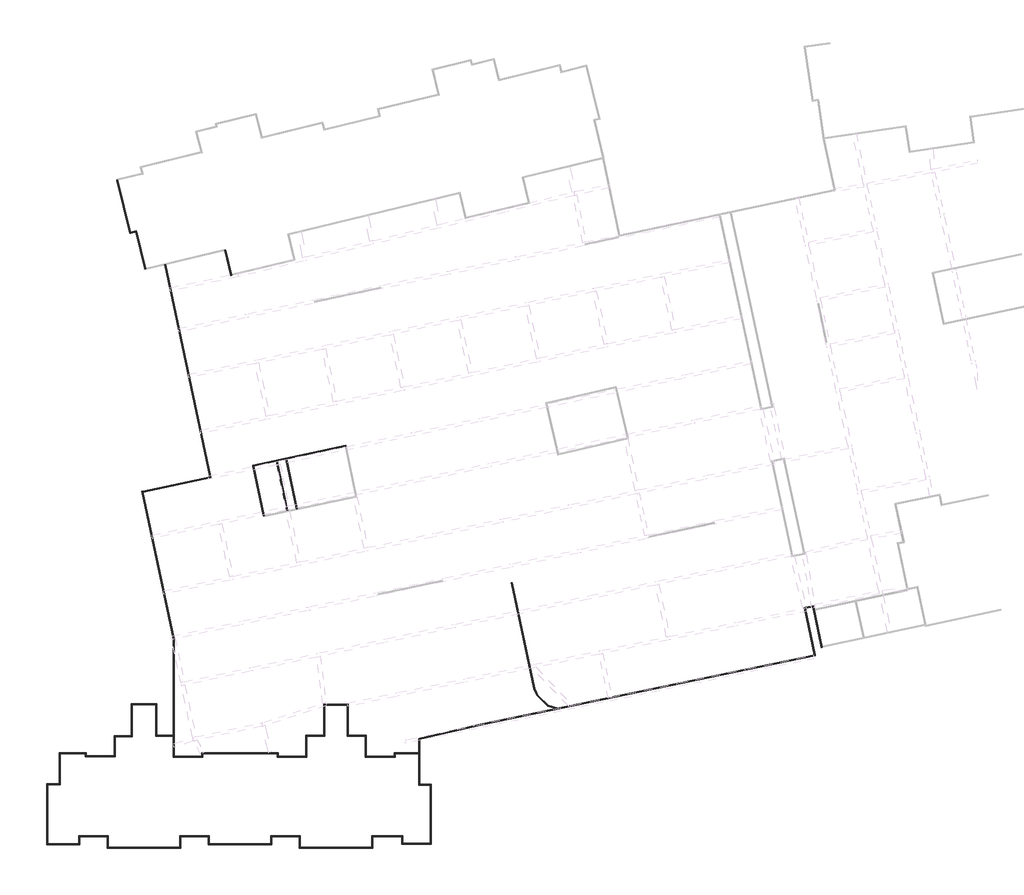
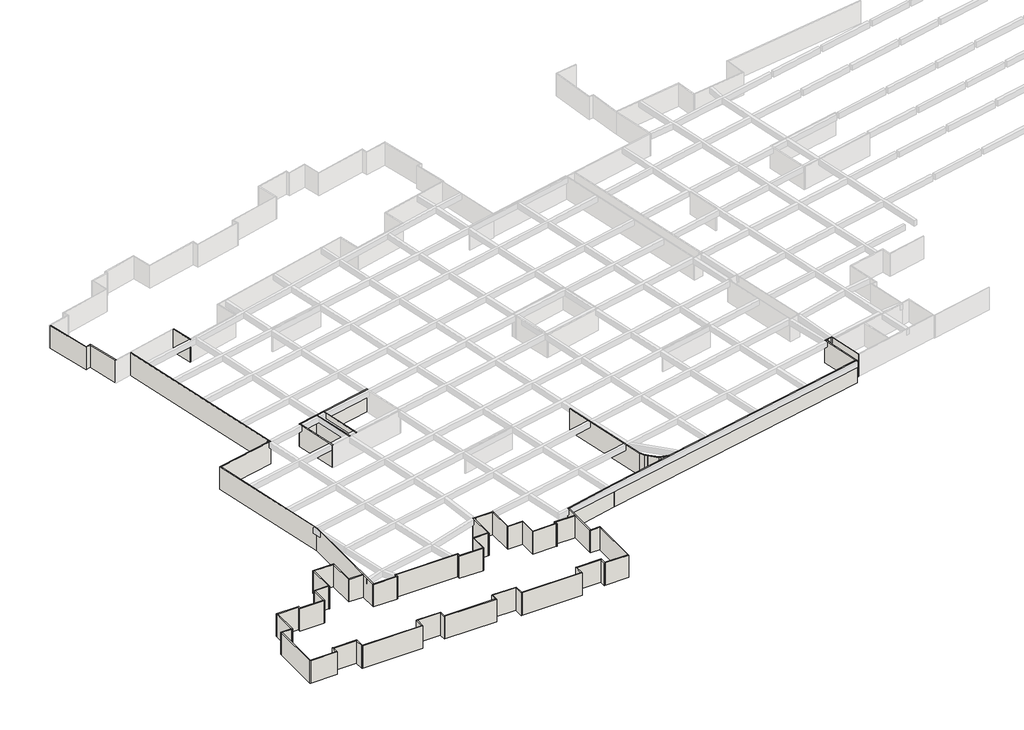
# One storey, part 1 of 14: 68 walls.
# Revit data of these elements (continued)
# Area, not placed, upper offset 0 mm, lower offset 0 mm
#   Number = "24"
#   Name = "fire_compart"
# Area, not placed, upper offset 0 mm, lower offset 0 mm
#   Number = "103"
#   Name = "main_building"
# Area, not placed, upper offset 0 mm, lower offset 0 mm
#   Number = "58"
#   Name = "fire_compart"
# Area, not placed, upper offset 0 mm, lower offset 0 mm
#   Number = "98"
#   Name = "fire_compart"
# Area, not placed, upper offset 0 mm, lower offset 0 mm
#   Number = "99"
#   Name = "main_building"
# Area, not placed, upper offset 0 mm, lower offset 0 mm
#   Number = "123"
#   Name = "main_building"
# Area at (-85290.668, -133064.536) mm, upper offset 0 mm, lower offset 0 mm
#   Number = "172"
#   Name = "fire_compart"
# Area, not placed, upper offset 0 mm, lower offset 0 mm
#   Number = "59"
#   Name = "fire_compart"
# Area at (-332558.106, -211971.491) mm, upper offset 0 mm, lower offset 0 mm
#   Number = "161"
#   Name = "main_building"
# Area at (-320626.882, -142375.996) mm, upper offset 0 mm, lower offset 0 mm
#   Number = "167"
#   Name = "main_building"
# Room, not placed, phase "新构造", upper offset 0 mm, lower offset 0 mm
#   Number = "1"
#   Name = "客餐厅"
# Room, not placed, phase "新构造", upper offset 0 mm, lower offset 0 mm
#   Number = "2"
#   Name = "阳台"
# Room, not placed, phase "新构造", upper offset 0 mm, lower offset 0 mm
#   Number = "3"
#   Name = "次卧"
# Room, not placed, phase "新构造", upper offset 0 mm, lower offset 0 mm
#   Number = "4"
#   Name = "厨房"
# Area, not placed, upper offset 0 mm, lower offset 0 mm
#   Number = "108"
#   Name = "main_building"
# Room, not placed, phase "新构造", upper offset 0 mm, lower offset 0 mm
#   Number = "5"
#   Name = "卫生间"
# Room, not placed, phase "新构造", upper offset 0 mm, lower offset 0 mm
#   Number = "6"
#   Name = "次卧"
# Room, not placed, phase "新构造", upper offset 0 mm, lower offset 0 mm
#   Number = "7"
#   Name = "主卧"
# Area, not placed, upper offset 0 mm, lower offset 0 mm
#   Number = "60"
#   Name = "fire_compart"
# Area, not placed, upper offset 0 mm, lower offset 0 mm
#   Number = "173"
#   Name = "面积"
# Area at (-58171.977, -181534.095) mm, upper offset 0 mm, lower offset 0 mm
#   Number = "174"
#   Name = "fire_compart"
# Area, not placed, upper offset 0 mm, lower offset 0 mm
#   Number = "23"
#   Name = "main_building"
# Area, not placed, upper offset 0 mm, lower offset 0 mm
#   Number = "124"
#   Name = "fire_compart"
# Area, not placed, upper offset 0 mm, lower offset 0 mm
#   Number = "36"
#   Name = "main_building"
# Area, not placed, upper offset 0 mm, lower offset 0 mm
#   Number = "37"
#   Name = "main_building"
# Area, not placed, upper offset 0 mm, lower offset 0 mm
#   Number = "38"
#   Name = "main_building"
# Area, not placed, upper offset 0 mm, lower offset 0 mm
#   Number = "39"
#   Name = "main_building"
# Area, not placed, upper offset 0 mm, lower offset 0 mm
#   Number = "40"
#   Name = "main_building"
# Area, not placed, upper offset 0 mm, lower offset 0 mm
#   Number = "64"
#   Name = "fire_compart"
# Area, not placed, upper offset 0 mm, lower offset 0 mm
#   Number = "61"
#   Name = "fire_compart"
# Area, not placed, upper offset 0 mm, lower offset 0 mm
#   Number = "65"
#   Name = "main_building"
# Area, not placed, upper offset 0 mm, lower offset 0 mm
#   Number = "104"
#   Name = "main_building"
# Area, not placed, upper offset 0 mm, lower offset 0 mm
#   Number = "62"
#   Name = "fire_compart"
# Area, not placed, upper offset 0 mm, lower offset 0 mm
#   Number = "125"
#   Name = "fire_compart"
# Area at (-54639.354, -203766.854) mm, upper offset 0 mm, lower offset 0 mm
#   Number = "164"
#   Name = "main_building"
# Area, not placed, upper offset 0 mm, lower offset 0 mm
#   Number = "63"
#   Name = "fire_compart"
# Area, not placed, upper offset 0 mm, lower offset 0 mm
#   Number = "66"
#   Name = "main_building"
# Area, not placed, upper offset 0 mm, lower offset 0 mm
#   Number = "126"
#   Name = "fire_compart"
# Area, not placed, upper offset 0 mm, lower offset 0 mm
#   Number = "83"
#   Name = "fire_compart"
# Area, not placed, upper offset 0 mm, lower offset 0 mm
#   Number = "84"
#   Name = "main_building"
# Area, not placed, upper offset 0 mm, lower offset 0 mm
#   Number = "150"
#   Name = "main_building"
# Area, not placed, upper offset 0 mm, lower offset 0 mm
#   Number = "127"
#   Name = "fire_compart"
# Area, not placed, upper offset 0 mm, lower offset 0 mm
#   Number = "7"
#   Name = "fire_compart_5"
# Area at (-166160.857, -117669.33) mm, upper offset 0 mm, lower offset 0 mm
#   Number = "175"
#   Name = "main_building"
# Area at (-77453.482, -110613.298) mm, upper offset 0 mm, lower offset 0 mm
#   Number = "176"
#   Name = "main_building"
# Area, not placed, upper offset 0 mm, lower offset 0 mm
#   Number = "128"
#   Name = "fire_compart"
# Area at (-242035.568, -186509.315) mm, upper offset 0 mm, lower offset 0 mm
#   Number = "162"
#   Name = "main_building"
# Area, not placed, upper offset 0 mm, lower offset 0 mm
#   Number = "129"
#   Name = "fire_compart"
# Area, not placed, upper offset 0 mm, lower offset 0 mm
#   Number = "151"
#   Name = "main_building"
# Area, not placed, upper offset 0 mm, lower offset 0 mm
#   Number = "130"
#   Name = "fire_compart"
# Area, not placed, upper offset 0 mm, lower offset 0 mm
#   Number = "109"
#   Name = "main_building"
# Area, not placed, upper offset 0 mm, lower offset 0 mm
#   Number = "67"
#   Name = "fire_compart"
# Area, not placed, upper offset 0 mm, lower offset 0 mm
#   Number = "112"
#   Name = "main_building"
# Area, not placed, upper offset 0 mm, lower offset 0 mm
#   Number = "131"
#   Name = "fire_compart"
# Area, not placed, upper offset 0 mm, lower offset 0 mm
#   Number = "68"
#   Name = "fire_compart"
# Area, not placed, upper offset 0 mm, lower offset 0 mm
#   Number = "152"
#   Name = "main_building"
# Area, not placed, upper offset 0 mm, lower offset 0 mm
#   Number = "132"
#   Name = "fire_compart"
# Area, not placed, upper offset 0 mm, lower offset 0 mm
#   Number = "1"
#   Name = "面积"
# Area, not placed, upper offset 0 mm, lower offset 0 mm
#   Number = "2"
#   Name = "防火区域1"
# Area, not placed, upper offset 0 mm, lower offset 0 mm
#   Number = "133"
#   Name = "fire_compart"
# Area, not placed, upper offset 0 mm, lower offset 0 mm
#   Number = "144"
#   Name = "fire_compart"
# Area, not placed, upper offset 0 mm, lower offset 0 mm
#   Number = "134"
#   Name = "fire_compart"
# Area, not placed, upper offset 0 mm, lower offset 0 mm
#   Number = "25"
#   Name = "fire_compart"
# Area, not placed, upper offset 0 mm, lower offset 0 mm
#   Number = "26"
#   Name = "fire_compart"
# Area, not placed, upper offset 0 mm, lower offset 0 mm
#   Number = "27"
#   Name = "fire_compart"
# Area, not placed, upper offset 0 mm, lower offset 0 mm
#   Number = "69"
#   Name = "fire_compart"
# Area, not placed, upper offset 0 mm, lower offset 0 mm
#   Number = "105"
#   Name = "main_building"
# Area, not placed, upper offset 0 mm, lower offset 0 mm
#   Number = "113"
#   Name = "main_building"
# Area, not placed, upper offset 0 mm, lower offset 0 mm
#   Number = "153"
#   Name = "main_building"
# Area, not placed, upper offset 0 mm, lower offset 0 mm
#   Number = "135"
#   Name = "fire_compart"
# Area, not placed, upper offset 0 mm, lower offset 0 mm
#   Number = "85"
#   Name = "fire_compart"
# Area, not placed, upper offset 0 mm, lower offset 0 mm
#   Number = "86"
#   Name = "main_building"
# Area, not placed, upper offset 0 mm, lower offset 0 mm
#   Number = "87"
#   Name = "main_building"
# Area, not placed, upper offset 0 mm, lower offset 0 mm
#   Number = "136"
#   Name = "fire_compart"
# Room, not placed, phase "新构造", upper offset 0 mm, lower offset 0 mm
#   Number = "8"
#   Name = "客餐厅"
# Area, not placed, upper offset 0 mm, lower offset 0 mm
#   Number = "70"
#   Name = "main_building"
# Area, not placed, upper offset 0 mm, lower offset 0 mm
#   Number = "156"
#   Name = "fire_compart"
# Area, not placed, upper offset 0 mm, lower offset 0 mm
#   Number = "154"
#   Name = "main_building"
# Area, not placed, upper offset 0 mm, lower offset 0 mm
#   Number = "114"
#   Name = "main_building"
# Area, not placed, upper offset 0 mm, lower offset 0 mm
#   Number = "8"
#   Name = "fire_compart_6"
# Area, not placed, upper offset 0 mm, lower offset 0 mm
#   Number = "137"
#   Name = "fire_compart"
# Area at (-165383.762, -173074.082) mm, upper offset 0 mm, lower offset 0 mm
#   Number = "163"
#   Name = "main_building"
# Area, not placed, upper offset 0 mm, lower offset 0 mm
#   Number = "138"
#   Name = "fire_compart"
# Area, not placed, upper offset 0 mm, lower offset 0 mm
#   Number = "3"
#   Name = "fire_compart_1"
# Area at (-296742.815, -161685.533) mm, upper offset 0 mm, lower offset 0 mm
#   Number = "168"
#   Name = "fire_compart"
# Area, not placed, upper offset 0 mm, lower offset 0 mm
#   Number = "139"
#   Name = "fire_compart"
# Area, not placed, upper offset 0 mm, lower offset 0 mm
#   Number = "71"
#   Name = "fire_compart"
# Room, not placed, phase "新构造", upper offset 0 mm, lower offset 0 mm
#   Number = "11"
#   Name = "房间"
# Area, not placed, upper offset 0 mm, lower offset 0 mm
#   Number = "140"
#   Name = "fire_compart"
# Area, not placed, upper offset 0 mm, lower offset 0 mm
#   Number = "155"
#   Name = "main_building"
# Area, not placed, upper offset 0 mm, lower offset 0 mm
#   Number = "106"
#   Name = "main_building"
# Room, not placed, phase "新构造", upper offset 0 mm, lower offset 0 mm
#   Number = "12"
#   Name = "房间"
# Area, not placed, upper offset 0 mm, lower offset 0 mm
#   Number = "110"
#   Name = "main_building"
# Area, not placed, upper offset 0 mm, lower offset 0 mm
#   Number = "115"
#   Name = "main_building"
# Area, not placed, upper offset 0 mm, lower offset 0 mm
#   Number = "141"
#   Name = "fire_compart"
# Area, not placed, upper offset 0 mm, lower offset 0 mm
#   Number = "100"
#   Name = "main_building"
# Room, not placed, phase "新构造", upper offset 0 mm, lower offset 0 mm
#   Number = "13"
#   Name = "房间"
# Room, not placed, phase "新构造", upper offset 0 mm, lower offset 0 mm
#   Number = "14"
#   Name = "房间"
# Area, not placed, upper offset 0 mm, lower offset 0 mm
#   Number = "72"
#   Name = "main_building"
# Room, not placed, phase "新构造", upper offset 0 mm, lower offset 0 mm
#   Number = "15"
#   Name = "房间"
# Area, not placed, upper offset 0 mm, lower offset 0 mm
#   Number = "88"
#   Name = "fire_compart"
# Room, not placed, phase "新构造", upper offset 0 mm, lower offset 0 mm
#   Number = "16"
#   Name = "房间"
# Area, not placed, upper offset 0 mm, lower offset 0 mm
#   Number = "28"
#   Name = "面积"
# Area, not placed, upper offset 0 mm, lower offset 0 mm
#   Number = "73"
#   Name = "fire_compart"
# Area, not placed, upper offset 0 mm, lower offset 0 mm
#   Number = "116"
#   Name = "main_building"
# Area, not placed, upper offset 0 mm, lower offset 0 mm
#   Number = "101"
#   Name = "main_building"
# Room, not placed, phase "新构造", upper offset 0 mm, lower offset 0 mm
#   Number = "17"
#   Name = "房间"
# Area, not placed, upper offset 0 mm, lower offset 0 mm
#   Number = "30"
#   Name = "main_building"
# Area, not placed, upper offset 0 mm, lower offset 0 mm
#   Number = "143"
#   Name = "fire_compart"
# Area, not placed, upper offset 0 mm, lower offset 0 mm
#   Number = "89"
#   Name = "main_building"
# Area, not placed, upper offset 0 mm, lower offset 0 mm
#   Number = "75"
#   Name = "main_building"
# Area, not placed, upper offset 0 mm, lower offset 0 mm
#   Number = "111"
#   Name = "main_building"
# Area, not placed, upper offset 0 mm, lower offset 0 mm
#   Number = "90"
#   Name = "fire_compart"
# Area, not placed, upper offset 0 mm, lower offset 0 mm
#   Number = "76"
#   Name = "main_building"
# Area, not placed, upper offset 0 mm, lower offset 0 mm
#   Number = "145"
#   Name = "fire_compart"
# Area, not placed, upper offset 0 mm, lower offset 0 mm
#   Number = "146"
#   Name = "fire_compart"
# Area, not placed, upper offset 0 mm, lower offset 0 mm
#   Number = "147"
#   Name = "fire_compart"
# Area, not placed, upper offset 0 mm, lower offset 0 mm
#   Number = "117"
#   Name = "main_building"
# Area, not placed, upper offset 0 mm, lower offset 0 mm
#   Number = "4"
#   Name = "fire_compart_2"
# Area, not placed, upper offset 0 mm, lower offset 0 mm
#   Number = "77"
#   Name = "main_building"
# Area, not placed, upper offset 0 mm, lower offset 0 mm
#   Number = "159"
#   Name = "fire_compart"
# Area, not placed, upper offset 0 mm, lower offset 0 mm
#   Number = "78"
#   Name = "main_building"
# Area, not placed, upper offset 0 mm, lower offset 0 mm
#   Number = "79"
#   Name = "main_building"
# Area, not placed, upper offset 0 mm, lower offset 0 mm
#   Number = "29"
#   Name = "main_building"
